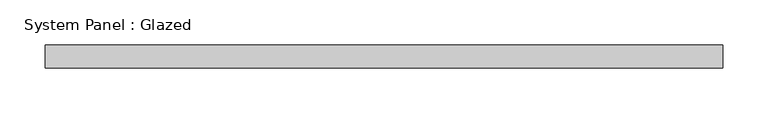
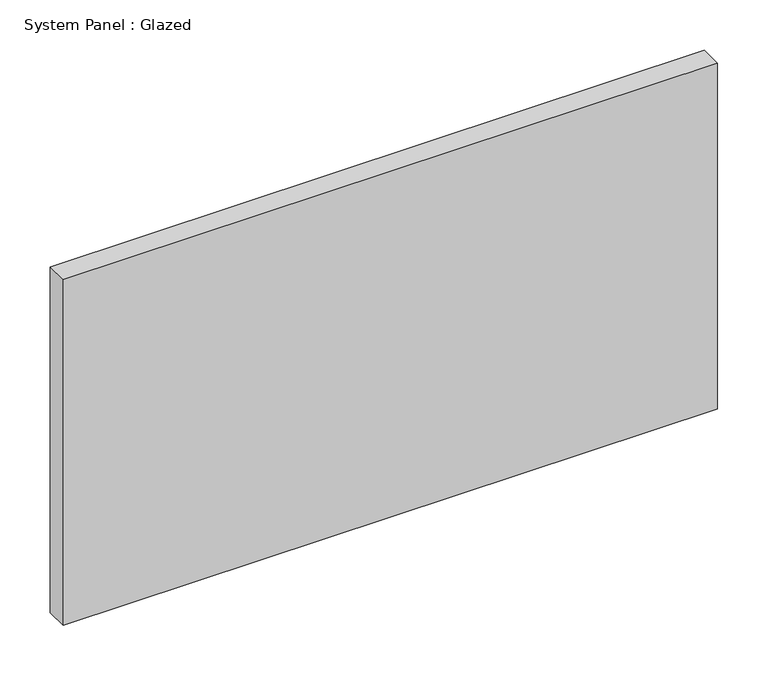
"""IFC4 building model written with IfcOpenShell, lengths in millimetres: plate geometry, System Panel : Glazed."""

from ifc_helpers import new_model, si_unit, origin, origin_with_axes, place, context, project, spatial, polyline, outline, extrude, source, transform, mapped, element, save


def system_panel_glazed_0122b756(model_context):
    return source(origin(), model_context, "Body", "SweptSolid", [
        extrude(outline(polyline([(374.8688463, 19.05), (-374.8688463, 19.05), (-374.8688463, 44.45), (374.8688463, 44.45), (374.8688463, 19.05)])), origin_with_axes(), (0.0, 0.0, 1.0), 419.1),
    ])


if __name__ == "__main__":
    model = new_model("IFC4")
    model_context = context("Model", 3, world=origin())
    ifc_project = project(units=[si_unit("LENGTHUNIT", "METRE", prefix="MILLI")], contexts=[model_context])
    site = spatial("IfcSite", under=ifc_project)
    building = spatial("IfcBuilding", under=site)
    placement = place(None, origin())
    system_panel_glazed_shape = system_panel_glazed_0122b756(model_context)
    element("IfcPlate", 1, ObjectType="System Panel : Glazed", at=placement, inside=building, context=model_context, shape_type="MappedRepresentation", body=[
        mapped(system_panel_glazed_shape, transform((0.0, 0.0, 0.0), x_axis=(1.0, 0.0, 0.0), y_axis=(0.0, 1.0, 0.0), z_axis=(0.0, 0.0, 1.0))),
    ])
    save(model, "model.ifc")

# Revit data of these elements
# Type "System Panel : Glazed"
#   Construction Type Id = "GSP4R"
#   Analytic Construction = "1/8 in Pilkington single glazing"
#   Visual Light Transmittance = 0.9
#   Solar Heat Gain Coefficient = 0.86
#   Heat Transfer Coefficient (U) = 1.18115 BTU/(h·ft²·°F)
#   Define Thermal Properties by = 1
# Element 1 (IfcPlate, "System Panel : Glazed")
#   Materials on its faces: "Glass"
# Materials
#   "Glass": class "Glass", colour RGB 0 128 192, transparency 0.75, Description = "Soda Lime Glass", Cost = 0
